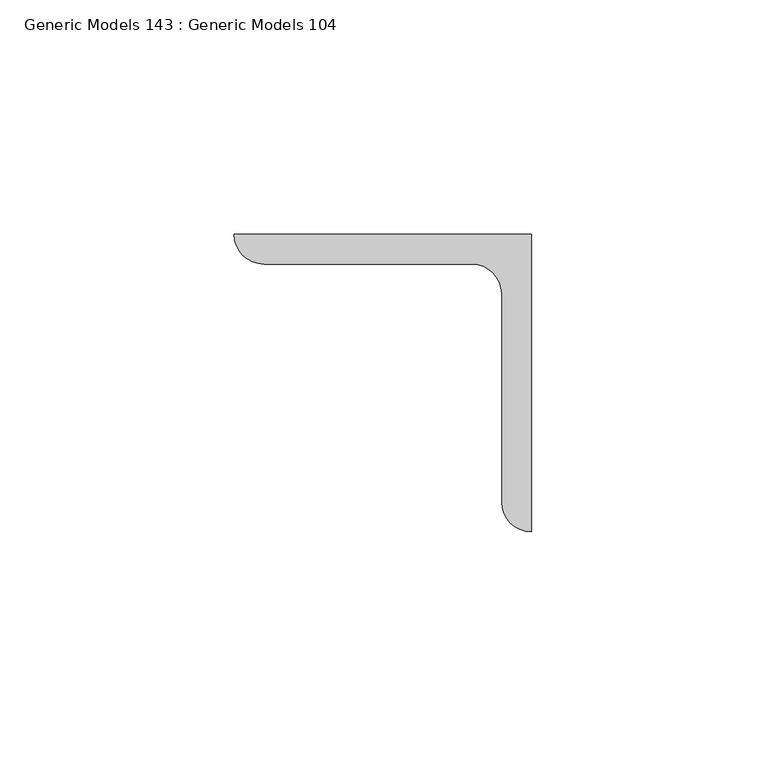
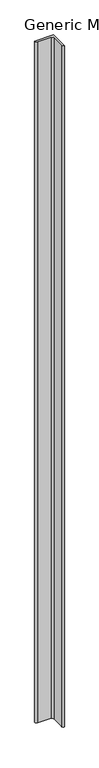
"""IFC4 building model written with IfcOpenShell, lengths in millimetres: proxy geometry, Generic Models 143 : Generic Models 104."""

from ifc_helpers import new_model, si_unit, point, frame, frame_2d, origin, place, context, project, spatial, polyline, circle_curve, trimmed, segment, composite_curve, outline, extrude, source, transform, mapped, element, save


def generic_models_143_generic_models_104_ef50b93d(model_context):
    return source(origin(), model_context, "Body", "SweptSolid", [
        extrude(outline(composite_curve([segment(polyline([(34421.7590778, 41071.1196612), (34421.7590778, 41007.6196612)]), True, "CONTINUOUS"), segment(trimmed(circle_curve(frame_2d((34421.7590778, 41013.9696612)), 6.35), [point((34421.7590778, 41007.6196612))], [point((34415.4090778, 41013.9696612))], False, "CARTESIAN"), True, "CONTINUOUS"), segment(polyline([(34415.4090778, 41013.9696612), (34415.4090778, 41058.4196612)]), True, "CONTINUOUS"), segment(trimmed(circle_curve(frame_2d((34409.0590778, 41058.4196612)), 6.35), [point((34415.4090778, 41058.4196612))], [point((34409.0590778, 41064.7696612))], True, "CARTESIAN"), True, "CONTINUOUS"), segment(polyline([(34409.0590778, 41064.7696612), (34364.6090778, 41064.7696612)]), True, "CONTINUOUS"), segment(trimmed(circle_curve(frame_2d((34364.6090778, 41071.1196612)), 6.35), [point((34364.6090778, 41064.7696612))], [point((34358.2590778, 41071.1196612))], False, "CARTESIAN"), True, "CONTINUOUS"), segment(polyline([(34358.2590778, 41071.1196612), (34421.7590778, 41071.1196612)]), True, "CONTINUOUS")], self_intersect=False)), frame((0.0, 0.0, 266407.9), z_axis=(0.0, 0.0, 1.0), x_axis=(1.0, 0.0, 0.0)), (0.0, 0.0, 1.0), 2432.1044757),
    ])


if __name__ == "__main__":
    model = new_model("IFC4")
    model_context = context("Model", 3, world=origin())
    ifc_project = project(units=[si_unit("LENGTHUNIT", "METRE", prefix="MILLI")], contexts=[model_context])
    site = spatial("IfcSite", under=ifc_project)
    building = spatial("IfcBuilding", under=site)
    placement = place(None, origin())
    generic_models_143_generic_models_104_shape = generic_models_143_generic_models_104_ef50b93d(model_context)
    element("IfcBuildingElementProxy", 1, Name="Generic Models 143 : Generic Models 104", ObjectType="Generic Models 143 : Generic Models 104", at=placement, inside=building, context=model_context, shape_type="MappedRepresentation", body=[
        mapped(generic_models_143_generic_models_104_shape, transform((0.0, 0.0, 0.0), x_axis=(1.0, 0.0, 0.0), y_axis=(0.0, 1.0, 0.0), z_axis=(0.0, 0.0, 1.0))),
    ])
    save(model, "model.ifc")

# Revit data of these elements
# Element 1 (IfcBuildingElementProxy, "Generic Models 143 : Generic Models 104")
#   Materials on its faces: "(2) BACK/BACK GALVANIZED ANGLES (2) L2 1/2 X 2 1/2 X 1/4\")"
# Materials
#   "(2) BACK/BACK GALVANIZED ANGLES (2) L2 1/2 X 2 1/2 X 1/4\")": class "Unassigned", colour RGB 211 211 211, transparency 0, Cost = 0
